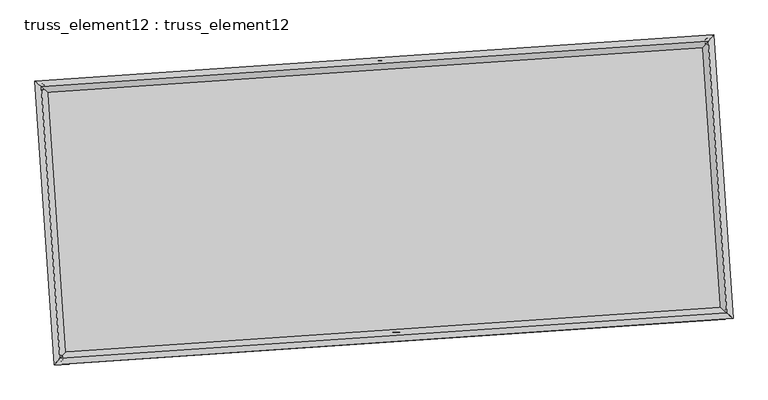
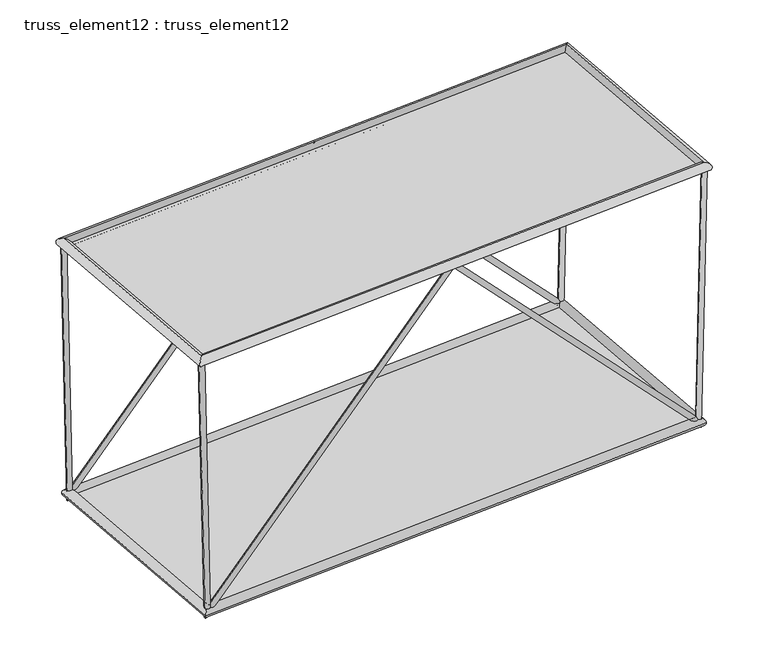
"""IFC4 building model written with IfcOpenShell, lengths in millimetres: plate geometry, truss_element12 : truss_element12."""

import ifcopenshell
import ifcopenshell.guid

model = None  # the IFC model being written
_history = None  # IfcOwnerHistory: only IFC2X3 demands one
_inside = {}  # id of a spatial element -> (the spatial element, [elements in it])
_under = {}  # id of a project, library or spatial element -> (it, [spatial elements below it])
_declared = {}  # id of a project -> (the project, [libraries it declares])
_typed = {}  # id of a type object -> (the type object, [elements of that type])
_made_of = {}  # id of a material, layer set ... -> (it, [elements and type objects made of it])


def new_model(schema):
    """Start an empty IFC model of exactly this schema.

    Asked for "IFC4X3", IfcOpenShell would pick the latest addendum, in which some entities
    have other attributes; the version numbers below select the first issue.
    IFC2X3 requires an IfcOwnerHistory on every rooted entity: one is made here for all.
    """
    global model, _history
    if schema == "IFC4X3":
        model = ifcopenshell.file(schema_version=(4, 3, 0, 0))
    else:
        model = ifcopenshell.file(schema=schema)
    _inside.clear()
    _under.clear()
    _declared.clear()
    _typed.clear()
    _made_of.clear()
    _history = None
    if model.schema == "IFC2X3":
        org = make("IfcOrganization", Name="unknown")
        user = make(
            "IfcPersonAndOrganization",
            ThePerson=make("IfcPerson", FamilyName="unknown"),
            TheOrganization=org,
        )
        app = make(
            "IfcApplication",
            ApplicationDeveloper=org,
            Version="unknown",
            ApplicationFullName="unknown",
            ApplicationIdentifier="unknown",
        )
        _history = make(
            "IfcOwnerHistory",
            OwningUser=user,
            OwningApplication=app,
            ChangeAction="ADDED",
            CreationDate=0,
        )
    return model


def make(cls, **values):
    """One entity of the class cls with the attributes given. An attribute that is None is left unset."""
    return model.create_entity(
        cls, **{name: value for name, value in values.items() if value is not None}
    )


def rooted(cls, **values):
    """An entity with a GlobalId (a new one), such as an element, a storey or a relation."""
    return make(cls, GlobalId=ifcopenshell.guid.new(), OwnerHistory=_history, **values)


def si_unit(unit_type, name, prefix=None):
    """IfcSIUnit, for example si_unit("LENGTHUNIT", "METRE", prefix="MILLI")."""
    return make("IfcSIUnit", UnitType=unit_type, Prefix=prefix, Name=name)


def assignment(units):
    """IfcUnitAssignment: the units of a project."""
    return None if units is None else make("IfcUnitAssignment", Units=units)


def point(xyz):
    """IfcCartesianPoint."""
    return None if xyz is None else make("IfcCartesianPoint", Coordinates=xyz)


def direction(xyz):
    """IfcDirection."""
    return None if xyz is None else make("IfcDirection", DirectionRatios=xyz)


def frame(location, z_axis=None, x_axis=None):
    """IfcAxis2Placement3D, a coordinate frame: its origin and axes. An axis left out is left unset."""
    return make(
        "IfcAxis2Placement3D",
        Location=point(location),
        Axis=direction(z_axis),
        RefDirection=direction(x_axis),
    )


def origin():
    """The frame at (0, 0, 0) with its axes left unset."""
    return frame((0.0, 0.0, 0.0))


def origin_with_axes():
    """The frame at (0, 0, 0) with the z axis (0, 0, 1) and the x axis (1, 0, 0) written out."""
    return frame((0.0, 0.0, 0.0), z_axis=(0.0, 0.0, 1.0), x_axis=(1.0, 0.0, 0.0))


def place(relative_to, where):
    """IfcLocalPlacement: puts the frame where relative to a parent placement (None: the world)."""
    return make(
        "IfcLocalPlacement", PlacementRelTo=relative_to, RelativePlacement=where
    )


def context(
    kind, dimensions, precision=None, world=None, true_north=None, identifier=None
):
    """IfcGeometricRepresentationContext, for example the 3D "Model" context."""
    return make(
        "IfcGeometricRepresentationContext",
        ContextIdentifier=identifier,
        ContextType=kind,
        CoordinateSpaceDimension=dimensions,
        Precision=precision,
        WorldCoordinateSystem=world,
        TrueNorth=true_north,
    )


def project(units=None, contexts=None):
    """IfcProject with its units and contexts."""
    return rooted(
        "IfcProject",
        Name="project",
        RepresentationContexts=contexts,
        UnitsInContext=assignment(units),
    )


def spatial(cls, under=None, at=None, **own):
    """A site, building, storey or space (cls), placed at a placement, below another one or the project."""
    s = rooted(cls, ObjectPlacement=at, **own)
    if under is not None:
        _under.setdefault(under.id(), (under, []))[1].append(s)
    return s


def polyline(points):
    """IfcPolyline through the points."""
    return make("IfcPolyline", Points=[point(p) for p in points])


def circle_curve(where, radius):
    """IfcCircle in the frame where."""
    return make("IfcCircle", Position=where, Radius=radius)


def ellipse_curve(where, semi_axis1, semi_axis2):
    """IfcEllipse in the frame where."""
    return make(
        "IfcEllipse", Position=where, SemiAxis1=semi_axis1, SemiAxis2=semi_axis2
    )


def outline(outer, holes=None, kind="AREA"):
    """IfcArbitraryClosedProfileDef: a profile drawn as a closed curve; with holes, ...WithVoids."""
    if holes is None:
        return make("IfcArbitraryClosedProfileDef", ProfileType=kind, OuterCurve=outer)
    return make(
        "IfcArbitraryProfileDefWithVoids",
        ProfileType=kind,
        OuterCurve=outer,
        InnerCurves=holes,
    )


def extrude(swept, where, along, depth):
    """IfcExtrudedAreaSolid: the profile swept, set in the frame where, extruded along a direction by depth."""
    return make(
        "IfcExtrudedAreaSolid",
        SweptArea=swept,
        Position=where,
        ExtrudedDirection=direction(along),
        Depth=depth,
    )


def shape(context_of_items, identifier, shape_type, items):
    """IfcShapeRepresentation: the items that make up one representation, for example the "Body"."""
    return make(
        "IfcShapeRepresentation",
        ContextOfItems=context_of_items,
        RepresentationIdentifier=identifier,
        RepresentationType=shape_type,
        Items=items,
    )


def source(mapping_origin, context_of_items, identifier, shape_type, items):
    """IfcRepresentationMap: a shape defined once, which mapped items show again and again."""
    return make(
        "IfcRepresentationMap",
        MappingOrigin=mapping_origin,
        MappedRepresentation=shape(context_of_items, identifier, shape_type, items),
    )


def transform(
    local_origin,
    x_axis=None,
    y_axis=None,
    z_axis=None,
    scale=None,
    scale2=None,
    scale3=None,
    uniform=True,
):
    """IfcCartesianTransformationOperator3D, or its non-uniform kind. x_axis, y_axis, z_axis: its Axis1, 2, 3."""
    if uniform:
        return make(
            "IfcCartesianTransformationOperator3D",
            Axis1=direction(x_axis),
            Axis2=direction(y_axis),
            LocalOrigin=point(local_origin),
            Scale=scale,
            Axis3=direction(z_axis),
        )
    return make(
        "IfcCartesianTransformationOperator3DnonUniform",
        Axis1=direction(x_axis),
        Axis2=direction(y_axis),
        LocalOrigin=point(local_origin),
        Scale=scale,
        Axis3=direction(z_axis),
        Scale2=scale2,
        Scale3=scale3,
    )


def mapped(mapping_source, mapping_target):
    """IfcMappedItem: shows the shape of a source again, moved by a transform."""
    return make(
        "IfcMappedItem", MappingSource=mapping_source, MappingTarget=mapping_target
    )


def made_of(thing, what):
    """Note that an element or type object is made of a material, layer set ...; save() writes the relation."""
    if what is not None:
        _made_of.setdefault(what.id(), (what, []))[1].append(thing)
    return thing


def element(
    cls,
    number,
    at=None,
    inside=None,
    cuts=None,
    type_object=None,
    material=None,
    context=None,
    identifier="Body",
    shape_type=None,
    held_by="IfcProductDefinitionShape",
    body=None,
    shapes=None,
    **own,
):
    """One element of the class cls, such as IfcWall. Its Tag is "e" and its number.

    at: its placement. inside: the storey or other place that contains it. cuts: it is an
    opening in that element (IfcRelVoidsElement). A single representation is given by context,
    identifier, shape_type and body (its items); several are given by shapes. held_by: the class
    of the entity that holds the representations. save() writes the other relations.
    """
    e = rooted(cls, Tag="e%d" % number, ObjectPlacement=at, **own)
    if body is not None:
        shapes = [shape(context, identifier, shape_type, body)]
    if shapes is not None:
        e.Representation = make(held_by, Representations=shapes)
    if inside is not None:
        _inside.setdefault(inside.id(), (inside, []))[1].append(e)
    if cuts is not None:
        rooted(
            "IfcRelVoidsElement", RelatingBuildingElement=cuts, RelatedOpeningElement=e
        )
    if type_object is not None:
        _typed.setdefault(type_object.id(), (type_object, []))[1].append(e)
    return made_of(e, material)


def aggregate(whole, parts):
    """IfcRelAggregates: a whole, such as a stair, and the parts it consists of."""
    return rooted("IfcRelAggregates", RelatingObject=whole, RelatedObjects=parts)


def save(model, path):
    """Write the relations noted so far, then the file.

    IfcRelAggregates (storeys below a building ...), IfcRelContainedInSpatialStructure (elements
    in a storey), IfcRelDefinesByType, IfcRelAssociatesMaterial and IfcRelDeclares: one each for
    every whole, place, type object, material and project.
    """
    for whole, parts in _under.values():
        aggregate(whole, parts)
    for where, things in _inside.values():
        rooted(
            "IfcRelContainedInSpatialStructure",
            RelatedElements=things,
            RelatingStructure=where,
        )
    for kind, things in _typed.values():
        rooted("IfcRelDefinesByType", RelatedObjects=things, RelatingType=kind)
    for what, things in _made_of.values():
        rooted("IfcRelAssociatesMaterial", RelatedObjects=things, RelatingMaterial=what)
    for by, libraries in _declared.values():
        rooted("IfcRelDeclares", RelatingContext=by, RelatedDefinitions=libraries)
    model.write(path)


def plane_surface(at):
    """IfcPlane: the flat surface through the origin of the frame at, square to its z axis."""
    return make("IfcPlane", Position=at)


def cylinder_surface(at, radius):
    """IfcCylindricalSurface: all points at the distance radius from the z axis of the frame at."""
    return make("IfcCylindricalSurface", Position=at, Radius=radius)


def advanced_brep(points, edges, surfaces, faces):
    """IfcAdvancedBrep: a solid bounded by faces that lie on surfaces and meet in shared edges.

    An edge is (start, end): straight between two places in points (the first is 0);
    or (start, end, curve); or (start, end, curve, False) where it runs against its curve.
    A face is (place in surfaces, loops), or (place, loops, False) where it looks against
    its surface's normal. A loop lists edges by number (the first is 1), with a minus sign
    where the edge is run from its end to its start. The first loop is the outer one.
    """
    corners = [point(p) for p in points]
    vertices = [make("IfcVertexPoint", VertexGeometry=c) for c in corners]
    made = []
    for start, end, *more in edges:
        made.append(
            make(
                "IfcEdgeCurve",
                EdgeStart=vertices[start],
                EdgeEnd=vertices[end],
                EdgeGeometry=more[0] if more else make("IfcPolyline", Points=[corners[start], corners[end]]),
                SameSense=more[1] if len(more) > 1 else True,
            )
        )
    hull = []
    for where, loops, *sense in faces:
        bounds = []
        for j, loop in enumerate(loops):
            ring = [make("IfcOrientedEdge", EdgeElement=made[abs(k) - 1], Orientation=k > 0) for k in loop]
            bounds.append(
                make(
                    "IfcFaceOuterBound" if j == 0 else "IfcFaceBound",
                    Bound=make("IfcEdgeLoop", EdgeList=ring),
                    Orientation=True,
                )
            )
        hull.append(make("IfcAdvancedFace", Bounds=bounds, FaceSurface=surfaces[where], SameSense=sense[0] if sense else True))
    return make("IfcAdvancedBrep", Outer=make("IfcClosedShell", CfsFaces=hull))


def truss_element12_truss_element12_d9043aa5(model_context):
    return source(origin(), model_context, "Body", "SolidModel", [
        advanced_brep(
        [(-3779.3847927, 2268.4205144, 4999.8287822), (-3878.4619663, 2255.0610807, 4997.5398535), (-3667.7051723, 2276.0355231, 121.2875859), (-3761.2817105, 2263.0511569, -121.2875859), (1064.0307623, 2598.6746095, 5070.7911995), (1064.4743138, 2592.1011158, 4926.5631841), (5795.1587841, 2921.2722446, 121.2833632), (5889.602193, 2921.1082439, -121.2833632), (5907.4418107, 2928.9283974, 4999.8207113), (6007.4151005, 2929.1414582, 4997.5194202)],
        [
            (0, 1, circle_curve(frame((-3828.9233795, 2261.7407976, 4998.6843179), z_axis=(-0.022885987621300542, -0.0015605084981128968, 0.9997368635715225), x_axis=(-0.1335949015683581, 0.9910348723202073, -0.0015113306095192321)), 50.0)),
            (1, 0, circle_curve(frame((-3828.9233795, 2261.7407976, 4998.6843179), z_axis=(-0.022885987621300542, -0.0015605084981128968, 0.9997368635715225), x_axis=(-0.1335949015683581, 0.9910348723202073, -0.0015113306095192321)), 50.0)),
            (0, 2),
            (2, 3, ellipse_curve(frame((-3714.4934414, 2269.54334, 0.0), z_axis=(-0.9299643254301769, -0.06341073222572768, 0.3621400729908157), x_axis=(0.36130113787628076, 0.024635751157578885, 0.9321236868217687)), 130.4029578, 50.0)),
            (3, 1),
            (3, 2, ellipse_curve(frame((-3714.4934414, 2269.54334, 0.0), z_axis=(-0.9299643254301769, -0.06341073222572768, 0.3621400729908157), x_axis=(0.36130113787628076, 0.024635751157578885, 0.9321236868217687)), 130.4029578, 50.0)),
            (2, 4),
            (4, 5, ellipse_curve(frame((1064.252538, 2595.3878627, 4998.6771918), z_axis=(-0.9976833955542866, -0.06802823819320543, 3.230475386038004e-05), x_axis=(-3.222991654096142e-05, -2.1976354914675906e-06, -0.9999999994782015)), 72.2710337, 50.0)),
            (5, 3),
            (5, 4, ellipse_curve(frame((1064.252538, 2595.3878627, 4998.6771918), z_axis=(-0.9976833955542866, -0.06802823819320543, 3.230475386038004e-05), x_axis=(-3.222991654096142e-05, -2.1976354914675906e-06, -0.9999999994782015)), 72.2710337, 50.0)),
            (4, 6),
            (6, 7, ellipse_curve(frame((5842.3804885, 2921.1902443, 0.0), z_axis=(-0.9299983802713416, -0.06341305429589221, -0.3620522023652769), x_axis=(-0.36121347081217786, -0.024629773473731513, 0.9321578207376972)), 130.3936428, 50.0)),
            (7, 5),
            (7, 6, ellipse_curve(frame((5842.3804885, 2921.1902443, 0.0), z_axis=(-0.9299983802713416, -0.06341305429589221, -0.3620522023652769), x_axis=(-0.36121347081217786, -0.024629773473731513, 0.9321578207376972)), 130.3936428, 50.0)),
            (8, 9, circle_curve(frame((5957.4284556, 2929.0349278, 4998.6700657), z_axis=(0.0230095934179778, 0.0015689367075186376, 0.9997340131496715), x_axis=(-0.002166147289386425, 0.9999964994670225, -0.001519493212205327)), 50.0)),
            (9, 8, circle_curve(frame((5957.4284556, 2929.0349278, 4998.6700657), z_axis=(0.0230095934179778, 0.0015689367075186376, 0.9997340131496715), x_axis=(-0.002166147289386425, 0.9999964994670225, -0.001519493212205327)), 50.0)),
            (6, 8),
            (9, 7),
        ],
        [
            plane_surface(frame((-3828.9233795, 2311.7407366, 4998.7623637), z_axis=(-0.022885987621301448, -0.0015605084981140727, 0.9997368635715226), x_axis=(0.9997380814846446, -3.572313472144376e-05, 0.02288595974085441))),
            cylinder_surface(frame((-3828.9233795, 2261.7407976, 4998.6843179), z_axis=(-0.022885987621300546, -0.0015605084981128972, 0.9997368635715227), x_axis=(-0.1335949015683581, 0.9910348723202073, -0.0015113306095192321)), 50.0),
            cylinder_surface(frame((-3714.4934414, 2269.54334, 0.0), z_axis=(-0.6902606627361213, -0.04706625066554751, -0.7220283827713277), x_axis=(-0.020420229147649776, 0.998751823015369, -0.045583004124724665)), 50.0),
            cylinder_surface(frame((1064.252538, 2595.3878627, 4998.6771918), z_axis=(-0.6902141194664037, -0.04706307705691311, 0.7220730822203193), x_axis=(-0.11534357052060634, 0.9922793612045488, -0.045579930529241086)), 50.0),
            plane_surface(frame((5957.4284556, 2879.0349894, 4998.7485334), z_axis=(0.023009593417979597, 0.0015689367075153572, 0.9997340131496715), x_axis=(0.9997352442575682, -3.611015610971435e-05, -0.023009565083185635))),
            cylinder_surface(frame((5842.3804885, 2921.1902443, 0.0), z_axis=(-0.023009593417977797, -0.0015689367075186372, -0.9997340131496713), x_axis=(-0.002166147289386425, 0.9999964994670225, -0.001519493212205327)), 50.0),
        ],
        [
            (0, [[1, 2]]),
            (1, [[-1, 3, 4, 5]]),
            (1, [[-2, -5, 6, -3]]),
            (2, [[-4, 7, 8, 9]]),
            (2, [[-6, -9, 10, -7]]),
            (3, [[-8, 11, 12, 13]]),
            (3, [[-10, -13, 14, -11]]),
            (4, [[15, 16]]),
            (5, [[-12, 17, -16, 18]]),
            (5, [[-14, -18, -15, -17]]),
        ],
    ),
        advanced_brep(
        [(-3507.2718398, -1722.3130699, 4999.8287822), (-3606.3490134, -1735.6725036, 4997.5398535), (-3395.5922194, -1714.6980612, 121.2875859), (-3489.1687576, -1727.6824274, -121.2875859), (1336.1437152, -1392.0589748, 5070.7911995), (1336.5872667, -1398.6324685, 4926.5631841), (6067.271737, -1069.4613397, 121.2833632), (6161.7151459, -1069.6253404, -121.2833632), (6179.5547636, -1061.8051869, 4999.8207113), (6279.5280534, -1061.5921261, 4997.5194202)],
        [
            (0, 1, circle_curve(frame((-3556.8104266, -1728.9927867, 4998.6843179), z_axis=(-0.022885987621300105, -0.0015605084981129068, 0.9997368635715226), x_axis=(-0.13359490156835802, 0.9910348723202074, -0.001511330609519162)), 50.0)),
            (1, 0, circle_curve(frame((-3556.8104266, -1728.9927867, 4998.6843179), z_axis=(-0.022885987621300105, -0.0015605084981129068, 0.9997368635715226), x_axis=(-0.13359490156835802, 0.9910348723202074, -0.001511330609519162)), 50.0)),
            (0, 2),
            (2, 3, ellipse_curve(frame((-3442.3804885, -1721.1902443, 0.0), z_axis=(-0.9299643254301768, -0.06341073222572771, 0.36214007299081585), x_axis=(0.3613011378762808, 0.024635751157578854, 0.9321236868217686)), 130.4029578, 50.0)),
            (3, 1),
            (3, 2, ellipse_curve(frame((-3442.3804885, -1721.1902443, 0.0), z_axis=(-0.9299643254301768, -0.06341073222572771, 0.36214007299081585), x_axis=(0.3613011378762808, 0.024635751157578854, 0.9321236868217686)), 130.4029578, 50.0)),
            (2, 4),
            (4, 5, ellipse_curve(frame((1336.3654909, -1395.3457216, 4998.6771918), z_axis=(-0.9976833955542866, -0.06802823819320533, 3.230475386021957e-05), x_axis=(-3.222991654080765e-05, -2.19763549153486e-06, -0.9999999994782015)), 72.2710337, 50.0)),
            (5, 3),
            (5, 4, ellipse_curve(frame((1336.3654909, -1395.3457216, 4998.6771918), z_axis=(-0.9976833955542866, -0.06802823819320533, 3.230475386021957e-05), x_axis=(-3.222991654080765e-05, -2.19763549153486e-06, -0.9999999994782015)), 72.2710337, 50.0)),
            (4, 6),
            (6, 7, ellipse_curve(frame((6114.4934414, -1069.54334, 0.0), z_axis=(-0.9299983802713416, -0.06341305429589225, -0.3620522023652771), x_axis=(-0.3612134708121779, -0.02462977347373136, 0.9321578207376972)), 130.3936428, 50.0)),
            (7, 5),
            (7, 6, ellipse_curve(frame((6114.4934414, -1069.54334, 0.0), z_axis=(-0.9299983802713416, -0.06341305429589225, -0.3620522023652771), x_axis=(-0.3612134708121779, -0.02462977347373136, 0.9321578207376972)), 130.3936428, 50.0)),
            (8, 9, circle_curve(frame((6229.5414085, -1061.6986565, 4998.6700657), z_axis=(0.023009593417977526, 0.0015689367075187803, 0.9997340131496715), x_axis=(-0.0021661472893863346, 0.9999964994670225, -0.0015194932122054722)), 50.0)),
            (9, 8, circle_curve(frame((6229.5414085, -1061.6986565, 4998.6700657), z_axis=(0.023009593417977526, 0.0015689367075187803, 0.9997340131496715), x_axis=(-0.0021661472893863346, 0.9999964994670225, -0.0015194932122054722)), 50.0)),
            (6, 8),
            (9, 7),
        ],
        [
            plane_surface(frame((-3556.8104266, -1678.9928477, 4998.7623637), z_axis=(-0.022885987621301448, -0.0015605084981140768, 0.9997368635715226), x_axis=(0.9997380814846446, -3.572313472144376e-05, 0.02288595974085441))),
            cylinder_surface(frame((-3556.8104266, -1728.9927867, 4998.6843179), z_axis=(-0.022885987621300105, -0.0015605084981129068, 0.9997368635715226), x_axis=(-0.13359490156835802, 0.9910348723202074, -0.001511330609519162)), 50.0),
            cylinder_surface(frame((-3442.3804885, -1721.1902443, 0.0), z_axis=(-0.6902606627361211, -0.04706625066554749, -0.722028382771328), x_axis=(-0.020420229147649727, 0.998751823015369, -0.04558300412472467)), 50.0),
            cylinder_surface(frame((1336.3654909, -1395.3457216, 4998.6771918), z_axis=(-0.6902141194664038, -0.04706307705691299, 0.7220730822203194), x_axis=(-0.11534357052060609, 0.992279361204549, -0.04557993052924103)), 50.0),
            plane_surface(frame((6229.5414085, -1111.6985949, 4998.7485334), z_axis=(0.023009593417976044, 0.0015689367075153572, 0.9997340131496715), x_axis=(0.9997352442575682, -3.611015610971435e-05, -0.023009565083182082))),
            cylinder_surface(frame((6114.4934414, -1069.54334, 0.0), z_axis=(-0.023009593417977522, -0.0015689367075187798, -0.9997340131496713), x_axis=(-0.0021661472893863346, 0.9999964994670225, -0.0015194932122054722)), 50.0),
        ],
        [
            (0, [[1, 2]]),
            (1, [[-1, 3, 4, 5]]),
            (1, [[-2, -5, 6, -3]]),
            (2, [[-4, 7, 8, 9]]),
            (2, [[-6, -9, 10, -7]]),
            (3, [[-8, 11, 12, 13]]),
            (3, [[-10, -13, 14, -11]]),
            (4, [[15, 16]]),
            (5, [[-12, 17, -16, 18]]),
            (5, [[-14, -18, -15, -17]]),
        ],
    ),
        advanced_brep(
        [(-3556.8141269, -1728.996888, 4908.6843179), (-3556.8067263, -1728.9886855, 5088.6843178), (-3828.9191567, 2261.7372366, 5088.6843178), (-3828.9276023, 2261.7443585, 4908.6843179), (5957.4250162, 2929.0308444, 5088.6700657), (5957.431895, 2929.0390112, 4908.6700658), (6229.5374466, -1061.6950777, 5088.6700657), (6229.5453704, -1061.7022353, 4908.6700658)],
        [
            (0, 1, ellipse_curve(frame((-3556.8104266, -1728.9927867, 4998.6843179), z_axis=(-0.7535719234047111, 0.6573654662781341, 1.0273917260532269e-06), x_axis=(-0.6573654662773387, -0.7535719234054049, 1.0273917260533834e-06)), 127.2792206, 90.0)),
            (1, 2),
            (2, 3, ellipse_curve(frame((-3828.9233795, 2261.7407976, 4998.6843179), z_axis=(-0.6573654662773385, -0.7535719234054051, 1.0273917260535286e-06), x_axis=(0.7535719234047112, -0.6573654662781339, -1.0273917260533723e-06)), 127.2792206, 90.0)),
            (3, 0),
            (1, 0, ellipse_curve(frame((-3556.8104266, -1728.9927867, 4998.6843179), z_axis=(-0.7535719234047111, 0.6573654662781341, 1.0273917260532269e-06), x_axis=(-0.6573654662773387, -0.7535719234054049, 1.0273917260533834e-06)), 127.2792206, 90.0)),
            (3, 2, ellipse_curve(frame((-3828.9233795, 2261.7407976, 4998.6843179), z_axis=(-0.6573654662773385, -0.7535719234054051, 1.0273917260535286e-06), x_axis=(0.7535719234047112, -0.6573654662781339, -1.0273917260533723e-06)), 127.2792206, 90.0)),
            (2, 4),
            (4, 5, ellipse_curve(frame((5957.4284556, 2929.0349278, 4998.6700657), z_axis=(-0.7535719234047108, 0.6573654662781345, 1.027391726053518e-06), x_axis=(-0.6573654662773392, -0.7535719234054046, 1.0273917260533831e-06)), 127.2792206, 90.0)),
            (5, 3),
            (5, 4, ellipse_curve(frame((5957.4284556, 2929.0349278, 4998.6700657), z_axis=(-0.7535719234047108, 0.6573654662781345, 1.027391726053518e-06), x_axis=(-0.6573654662773392, -0.7535719234054046, 1.0273917260533831e-06)), 127.2792206, 90.0)),
            (4, 6),
            (6, 7, ellipse_curve(frame((6229.5414085, -1061.6986565, 4998.6700657), z_axis=(0.657365466277339, 0.7535719234054045, -1.0273917260532377e-06), x_axis=(-0.7535719234047105, 0.6573654662781346, 1.0273917260533721e-06)), 127.2792206, 90.0)),
            (7, 5),
            (7, 6, ellipse_curve(frame((6229.5414085, -1061.6986565, 4998.6700657), z_axis=(0.657365466277339, 0.7535719234054045, -1.0273917260532377e-06), x_axis=(-0.7535719234047105, 0.6573654662781346, 1.0273917260533721e-06)), 127.2792206, 90.0)),
            (6, 1),
            (0, 7),
        ],
        [
            cylinder_surface(frame((-3556.8104266, -1728.9927867, 4998.6843179), z_axis=(0.06802823822869865, -0.9976833960748769, 0.0), x_axis=(-0.9976833951038622, -0.06802823816248885, 4.411959662306044e-05)), 90.0),
            cylinder_surface(frame((-3828.9233795, 2261.7407976, 4998.6843179), z_axis=(-0.9976833960738238, -0.06802823822862583, 1.4529513128546934e-06), x_axis=(-0.06802823810492795, 0.9976833951709815, 4.266664531152834e-05)), 90.0),
            cylinder_surface(frame((5957.4284556, 2929.0349278, 4998.6700657), z_axis=(-0.06802823822869723, 0.9976833960748768, 0.0), x_axis=(0.99768339522756, 0.06802823817092192, 4.121369399999627e-05)), 90.0),
            cylinder_surface(frame((6229.5414085, -1061.6986565, 4998.6700657), z_axis=(0.9976833960738238, 0.0680282382286254, -1.452951312854488e-06), x_axis=(0.0680282382286254, -0.997683395162547, 4.2666645311528356e-05)), 90.0),
        ],
        [
            (0, [[1, 2, 3, 4]]),
            (0, [[5, -4, 6, -2]]),
            (1, [[-3, 7, 8, 9]]),
            (1, [[-6, -9, 10, -7]]),
            (2, [[-8, 11, 12, 13]]),
            (2, [[-10, -13, 14, -11]]),
            (3, [[-12, 15, -1, 16]]),
            (3, [[-14, -16, -5, -15]]),
        ],
    ),
        advanced_brep(
        [(-3358.7115243, -1625.2761972, 0.0), (-3526.0494527, -1817.1042913, 0.0), (-3810.4074885, 2353.2123043, 0.0), (-3618.5793943, 2185.8743758, 0.0), (5926.0494527, 3017.1042913, 0.0), (5758.7115243, 2825.2761972, 0.0), (6210.4074885, -1153.2123043, 0.0), (6018.5793943, -985.8743758, 0.0)],
        [
            (0, 1, ellipse_curve(frame((-3442.3804885, -1721.1902443, 0.0), z_axis=(-0.7535719234054589, 0.6573654662780799, 0.0), x_axis=(-0.65736546627808, -0.7535719234054586, 0.0)), 127.2792206, 90.0)),
            (1, 2),
            (2, 3, ellipse_curve(frame((-3714.4934414, 2269.54334, 0.0), z_axis=(-0.6573654662780799, -0.7535719234054586, 0.0), x_axis=(0.7535719234054586, -0.6573654662780801, 0.0)), 127.2792206, 90.0)),
            (3, 0),
            (1, 0, ellipse_curve(frame((-3442.3804885, -1721.1902443, 0.0), z_axis=(-0.7535719234054589, 0.6573654662780799, 0.0), x_axis=(-0.65736546627808, -0.7535719234054586, 0.0)), 127.2792206, 90.0)),
            (3, 2, ellipse_curve(frame((-3714.4934414, 2269.54334, 0.0), z_axis=(-0.6573654662780799, -0.7535719234054586, 0.0), x_axis=(0.7535719234054586, -0.6573654662780801, 0.0)), 127.2792206, 90.0)),
            (2, 4),
            (4, 5, ellipse_curve(frame((5842.3804885, 2921.1902443, 0.0), z_axis=(-0.7535719234054585, 0.6573654662780801, 0.0), x_axis=(-0.6573654662780801, -0.7535719234054586, 0.0)), 127.2792206, 90.0)),
            (5, 3),
            (5, 4, ellipse_curve(frame((5842.3804885, 2921.1902443, 0.0), z_axis=(-0.7535719234054585, 0.6573654662780801, 0.0), x_axis=(-0.6573654662780801, -0.7535719234054586, 0.0)), 127.2792206, 90.0)),
            (4, 6),
            (6, 7, ellipse_curve(frame((6114.4934414, -1069.54334, 0.0), z_axis=(0.65736546627808, 0.7535719234054584, 0.0), x_axis=(-0.7535719234054583, 0.6573654662780803, 0.0)), 127.2792206, 90.0)),
            (7, 5),
            (7, 6, ellipse_curve(frame((6114.4934414, -1069.54334, 0.0), z_axis=(0.65736546627808, 0.7535719234054584, 0.0), x_axis=(-0.7535719234054583, 0.6573654662780803, 0.0)), 127.2792206, 90.0)),
            (6, 1),
            (0, 7),
        ],
        [
            cylinder_surface(frame((-3442.3804885, -1721.1902443, 0.0), z_axis=(0.0680282382287028, -0.9976833960748764, 0.0), x_axis=(-0.9976833960748764, -0.0680282382287028, 0.0)), 90.0),
            cylinder_surface(frame((-3714.4934414, 2269.54334, 0.0), z_axis=(-0.9976833960748765, -0.06802823822870228, 0.0), x_axis=(-0.06802823822870228, 0.9976833960748765, 0.0)), 90.0),
            cylinder_surface(frame((5842.3804885, 2921.1902443, 0.0), z_axis=(-0.06802823822870217, 0.9976833960748765, 0.0), x_axis=(0.9976833960748765, 0.06802823822870217, 0.0)), 90.0),
            cylinder_surface(frame((6114.4934414, -1069.54334, 0.0), z_axis=(0.9976833960748765, 0.06802823822870213, 0.0), x_axis=(0.06802823822870213, -0.9976833960748765, 0.0)), 90.0),
        ],
        [
            (0, [[1, 2, 3, 4]]),
            (0, [[5, -4, 6, -2]]),
            (1, [[-3, 7, 8, 9]]),
            (1, [[-6, -9, 10, -7]]),
            (2, [[-8, 11, 12, 13]]),
            (2, [[-10, -13, 14, -11]]),
            (3, [[-12, 15, -1, 16]]),
            (3, [[-14, -16, -5, -15]]),
        ],
    ),
        extrude(outline(polyline([(-3442.3804885, -1721.1902443), (-3714.4934414, 2269.54334), (5842.3804885, 2921.1902443), (6114.4934414, -1069.54334), (-3442.3804885, -1721.1902443)])), origin_with_axes(), (0.0, 0.0, 1.0), 20.0),
        extrude(outline(polyline([(-1999.9999999, 4904.5377891), (2000.0000001, 4904.537789), (2000.0, -4904.5377891), (-2000.0, -4904.537789), (-1999.9999999, 4904.5377891)])), frame((1200.3090145, 600.0210705, 4998.6771918), z_axis=(1.4495854001402175e-06, 9.884171804557912e-08, 0.9999999999989445), x_axis=(-0.06802823822870323, 0.9976833960748764, 0.0)), (0.0, 0.0, 1.0), 20.0),
    ])


if __name__ == "__main__":
    model = new_model("IFC4")
    model_context = context("Model", 3, world=origin())
    ifc_project = project(units=[si_unit("LENGTHUNIT", "METRE", prefix="MILLI")], contexts=[model_context])
    site = spatial("IfcSite", under=ifc_project)
    building = spatial("IfcBuilding", under=site)
    placement = place(None, origin())
    truss_element12_truss_element12_shape = truss_element12_truss_element12_d9043aa5(model_context)
    element("IfcPlate", 1, ObjectType="truss_element12 : truss_element12", at=placement, inside=building, context=model_context, shape_type="MappedRepresentation", body=[
        mapped(truss_element12_truss_element12_shape, transform((0.0, 0.0, 0.0), x_axis=(1.0, 0.0, 0.0), y_axis=(0.0, 1.0, 0.0), z_axis=(0.0, 0.0, 1.0))),
    ])
    save(model, "model.ifc")

# Revit data of these elements
# Type "truss_element12 : truss_element12"
#   steellbar1 = 90 mm
#   steelbar2 = 50 mm
#   offset1 = 5000 mm
#   M = Default Roof
# Element 1 (IfcPlate, "truss_element12 : truss_element12")
#   Materials on its faces: "Default Roof"
# Materials
#   "Default Roof": class "Miscellaneous", colour RGB 0 127 0, transparency 0, Comments = "Rendering appearance not upgraded Rendering appearance not upgraded ", Cost = 0
